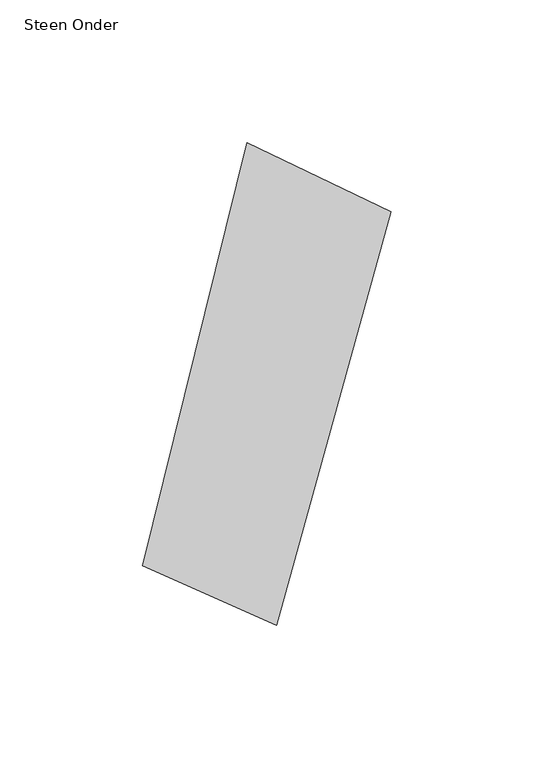
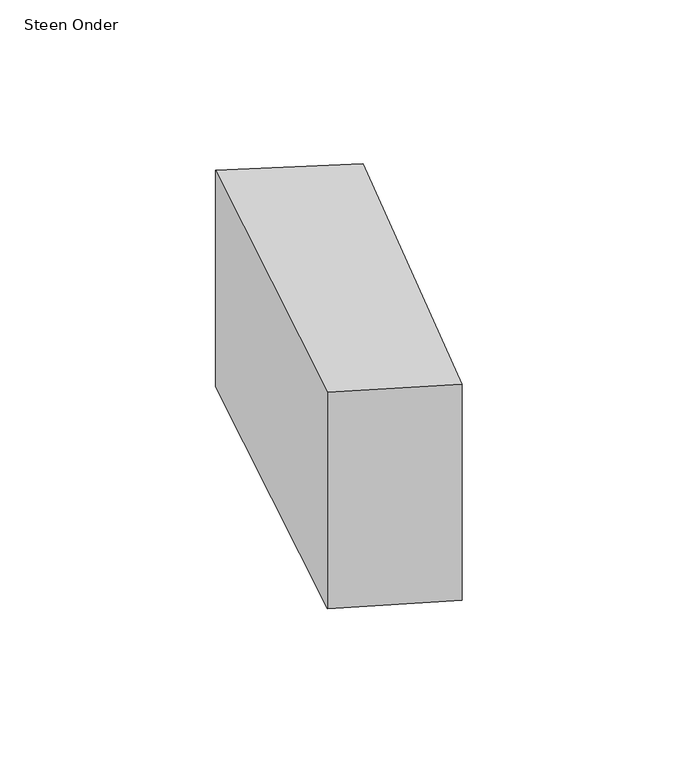
"""IFC4 building model written with IfcOpenShell, lengths in millimetres: proxy geometry, 00_GMA_steen_versie_4 : Steen Onder."""

import ifcopenshell
import ifcopenshell.guid

model = None  # the IFC model being written
_history = None  # IfcOwnerHistory: only IFC2X3 demands one
_inside = {}  # id of a spatial element -> (the spatial element, [elements in it])
_under = {}  # id of a project, library or spatial element -> (it, [spatial elements below it])
_declared = {}  # id of a project -> (the project, [libraries it declares])
_typed = {}  # id of a type object -> (the type object, [elements of that type])
_made_of = {}  # id of a material, layer set ... -> (it, [elements and type objects made of it])


def new_model(schema):
    """Start an empty IFC model of exactly this schema.

    Asked for "IFC4X3", IfcOpenShell would pick the latest addendum, in which some entities
    have other attributes; the version numbers below select the first issue.
    IFC2X3 requires an IfcOwnerHistory on every rooted entity: one is made here for all.
    """
    global model, _history
    if schema == "IFC4X3":
        model = ifcopenshell.file(schema_version=(4, 3, 0, 0))
    else:
        model = ifcopenshell.file(schema=schema)
    _inside.clear()
    _under.clear()
    _declared.clear()
    _typed.clear()
    _made_of.clear()
    _history = None
    if model.schema == "IFC2X3":
        org = make("IfcOrganization", Name="unknown")
        user = make(
            "IfcPersonAndOrganization",
            ThePerson=make("IfcPerson", FamilyName="unknown"),
            TheOrganization=org,
        )
        app = make(
            "IfcApplication",
            ApplicationDeveloper=org,
            Version="unknown",
            ApplicationFullName="unknown",
            ApplicationIdentifier="unknown",
        )
        _history = make(
            "IfcOwnerHistory",
            OwningUser=user,
            OwningApplication=app,
            ChangeAction="ADDED",
            CreationDate=0,
        )
    return model


def make(cls, **values):
    """One entity of the class cls with the attributes given. An attribute that is None is left unset."""
    return model.create_entity(
        cls, **{name: value for name, value in values.items() if value is not None}
    )


def rooted(cls, **values):
    """An entity with a GlobalId (a new one), such as an element, a storey or a relation."""
    return make(cls, GlobalId=ifcopenshell.guid.new(), OwnerHistory=_history, **values)


def si_unit(unit_type, name, prefix=None):
    """IfcSIUnit, for example si_unit("LENGTHUNIT", "METRE", prefix="MILLI")."""
    return make("IfcSIUnit", UnitType=unit_type, Prefix=prefix, Name=name)


def assignment(units):
    """IfcUnitAssignment: the units of a project."""
    return None if units is None else make("IfcUnitAssignment", Units=units)


def point(xyz):
    """IfcCartesianPoint."""
    return None if xyz is None else make("IfcCartesianPoint", Coordinates=xyz)


def direction(xyz):
    """IfcDirection."""
    return None if xyz is None else make("IfcDirection", DirectionRatios=xyz)


def frame(location, z_axis=None, x_axis=None):
    """IfcAxis2Placement3D, a coordinate frame: its origin and axes. An axis left out is left unset."""
    return make(
        "IfcAxis2Placement3D",
        Location=point(location),
        Axis=direction(z_axis),
        RefDirection=direction(x_axis),
    )


def origin():
    """The frame at (0, 0, 0) with its axes left unset."""
    return frame((0.0, 0.0, 0.0))


def origin_with_axes():
    """The frame at (0, 0, 0) with the z axis (0, 0, 1) and the x axis (1, 0, 0) written out."""
    return frame((0.0, 0.0, 0.0), z_axis=(0.0, 0.0, 1.0), x_axis=(1.0, 0.0, 0.0))


def place(relative_to, where):
    """IfcLocalPlacement: puts the frame where relative to a parent placement (None: the world)."""
    return make(
        "IfcLocalPlacement", PlacementRelTo=relative_to, RelativePlacement=where
    )


def context(
    kind, dimensions, precision=None, world=None, true_north=None, identifier=None
):
    """IfcGeometricRepresentationContext, for example the 3D "Model" context."""
    return make(
        "IfcGeometricRepresentationContext",
        ContextIdentifier=identifier,
        ContextType=kind,
        CoordinateSpaceDimension=dimensions,
        Precision=precision,
        WorldCoordinateSystem=world,
        TrueNorth=true_north,
    )


def project(units=None, contexts=None):
    """IfcProject with its units and contexts."""
    return rooted(
        "IfcProject",
        Name="project",
        RepresentationContexts=contexts,
        UnitsInContext=assignment(units),
    )


def spatial(cls, under=None, at=None, **own):
    """A site, building, storey or space (cls), placed at a placement, below another one or the project."""
    s = rooted(cls, ObjectPlacement=at, **own)
    if under is not None:
        _under.setdefault(under.id(), (under, []))[1].append(s)
    return s


def polyline(points):
    """IfcPolyline through the points."""
    return make("IfcPolyline", Points=[point(p) for p in points])


def outline(outer, holes=None, kind="AREA"):
    """IfcArbitraryClosedProfileDef: a profile drawn as a closed curve; with holes, ...WithVoids."""
    if holes is None:
        return make("IfcArbitraryClosedProfileDef", ProfileType=kind, OuterCurve=outer)
    return make(
        "IfcArbitraryProfileDefWithVoids",
        ProfileType=kind,
        OuterCurve=outer,
        InnerCurves=holes,
    )


def extrude(swept, where, along, depth):
    """IfcExtrudedAreaSolid: the profile swept, set in the frame where, extruded along a direction by depth."""
    return make(
        "IfcExtrudedAreaSolid",
        SweptArea=swept,
        Position=where,
        ExtrudedDirection=direction(along),
        Depth=depth,
    )


def shape(context_of_items, identifier, shape_type, items):
    """IfcShapeRepresentation: the items that make up one representation, for example the "Body"."""
    return make(
        "IfcShapeRepresentation",
        ContextOfItems=context_of_items,
        RepresentationIdentifier=identifier,
        RepresentationType=shape_type,
        Items=items,
    )


def source(mapping_origin, context_of_items, identifier, shape_type, items):
    """IfcRepresentationMap: a shape defined once, which mapped items show again and again."""
    return make(
        "IfcRepresentationMap",
        MappingOrigin=mapping_origin,
        MappedRepresentation=shape(context_of_items, identifier, shape_type, items),
    )


def transform(
    local_origin,
    x_axis=None,
    y_axis=None,
    z_axis=None,
    scale=None,
    scale2=None,
    scale3=None,
    uniform=True,
):
    """IfcCartesianTransformationOperator3D, or its non-uniform kind. x_axis, y_axis, z_axis: its Axis1, 2, 3."""
    if uniform:
        return make(
            "IfcCartesianTransformationOperator3D",
            Axis1=direction(x_axis),
            Axis2=direction(y_axis),
            LocalOrigin=point(local_origin),
            Scale=scale,
            Axis3=direction(z_axis),
        )
    return make(
        "IfcCartesianTransformationOperator3DnonUniform",
        Axis1=direction(x_axis),
        Axis2=direction(y_axis),
        LocalOrigin=point(local_origin),
        Scale=scale,
        Axis3=direction(z_axis),
        Scale2=scale2,
        Scale3=scale3,
    )


def mapped(mapping_source, mapping_target):
    """IfcMappedItem: shows the shape of a source again, moved by a transform."""
    return make(
        "IfcMappedItem", MappingSource=mapping_source, MappingTarget=mapping_target
    )


def made_of(thing, what):
    """Note that an element or type object is made of a material, layer set ...; save() writes the relation."""
    if what is not None:
        _made_of.setdefault(what.id(), (what, []))[1].append(thing)
    return thing


def element(
    cls,
    number,
    at=None,
    inside=None,
    cuts=None,
    type_object=None,
    material=None,
    context=None,
    identifier="Body",
    shape_type=None,
    held_by="IfcProductDefinitionShape",
    body=None,
    shapes=None,
    **own,
):
    """One element of the class cls, such as IfcWall. Its Tag is "e" and its number.

    at: its placement. inside: the storey or other place that contains it. cuts: it is an
    opening in that element (IfcRelVoidsElement). A single representation is given by context,
    identifier, shape_type and body (its items); several are given by shapes. held_by: the class
    of the entity that holds the representations. save() writes the other relations.
    """
    e = rooted(cls, Tag="e%d" % number, ObjectPlacement=at, **own)
    if body is not None:
        shapes = [shape(context, identifier, shape_type, body)]
    if shapes is not None:
        e.Representation = make(held_by, Representations=shapes)
    if inside is not None:
        _inside.setdefault(inside.id(), (inside, []))[1].append(e)
    if cuts is not None:
        rooted(
            "IfcRelVoidsElement", RelatingBuildingElement=cuts, RelatedOpeningElement=e
        )
    if type_object is not None:
        _typed.setdefault(type_object.id(), (type_object, []))[1].append(e)
    return made_of(e, material)


def aggregate(whole, parts):
    """IfcRelAggregates: a whole, such as a stair, and the parts it consists of."""
    return rooted("IfcRelAggregates", RelatingObject=whole, RelatedObjects=parts)


def save(model, path):
    """Write the relations noted so far, then the file.

    IfcRelAggregates (storeys below a building ...), IfcRelContainedInSpatialStructure (elements
    in a storey), IfcRelDefinesByType, IfcRelAssociatesMaterial and IfcRelDeclares: one each for
    every whole, place, type object, material and project.
    """
    for whole, parts in _under.values():
        aggregate(whole, parts)
    for where, things in _inside.values():
        rooted(
            "IfcRelContainedInSpatialStructure",
            RelatedElements=things,
            RelatingStructure=where,
        )
    for kind, things in _typed.values():
        rooted("IfcRelDefinesByType", RelatedObjects=things, RelatingType=kind)
    for what, things in _made_of.values():
        rooted("IfcRelAssociatesMaterial", RelatedObjects=things, RelatingMaterial=what)
    for by, libraries in _declared.values():
        rooted("IfcRelDeclares", RelatingContext=by, RelatedDefinitions=libraries)
    model.write(path)


def steen_onder_84ae347e(model_context):
    return source(origin(), model_context, "Body", "SweptSolid", [
        extrude(outline(polyline([(120.4860713, 140.7369891), (80.2413573, -4.0871159), (33.3347144, 16.6686862), (69.9199367, 164.9526815), (120.4860713, 140.7369891)])), origin_with_axes(), (0.0, 0.0, 1.0), 100.0),
    ])


if __name__ == "__main__":
    model = new_model("IFC4")
    model_context = context("Model", 3, world=origin())
    ifc_project = project(units=[si_unit("LENGTHUNIT", "METRE", prefix="MILLI")], contexts=[model_context])
    site = spatial("IfcSite", under=ifc_project)
    building = spatial("IfcBuilding", under=site)
    placement = place(None, origin())
    steen_onder_shape = steen_onder_84ae347e(model_context)
    element("IfcBuildingElementProxy", 1, Name="00_GMA_steen_versie_4 : Steen Onder", ObjectType="00_GMA_steen_versie_4 : Steen Onder", at=placement, inside=building, context=model_context, shape_type="MappedRepresentation", body=[
        mapped(steen_onder_shape, transform((0.0, 0.0, 0.0), x_axis=(1.0, 0.0, 0.0), y_axis=(0.0, 1.0, 0.0), z_axis=(0.0, 0.0, 1.0))),
    ])
    save(model, "model.ifc")

# Revit data of these elements
# Type "00_GMA_steen_versie_4 : Steen Onder"
#   StootVoegHalfBoven [instance default] = 5 mm
#   StootVoegHalf [instance default] = 5 mm
#   StootVoegBreedteOnder = 10 mm
#   StootVoegBreedteBoven = 10 mm
#   Steendikte = 100 mm
#   LintVoegOnderHalf = 0 mm
#   LintVoegOnder = 0 mm
#   LintVoegBovenHalf = 5 mm
#   LintVoegBoven = 10 mm
#   materiaal = none
#   MateriaalVoeg = none
#   Default Elevation = 0
